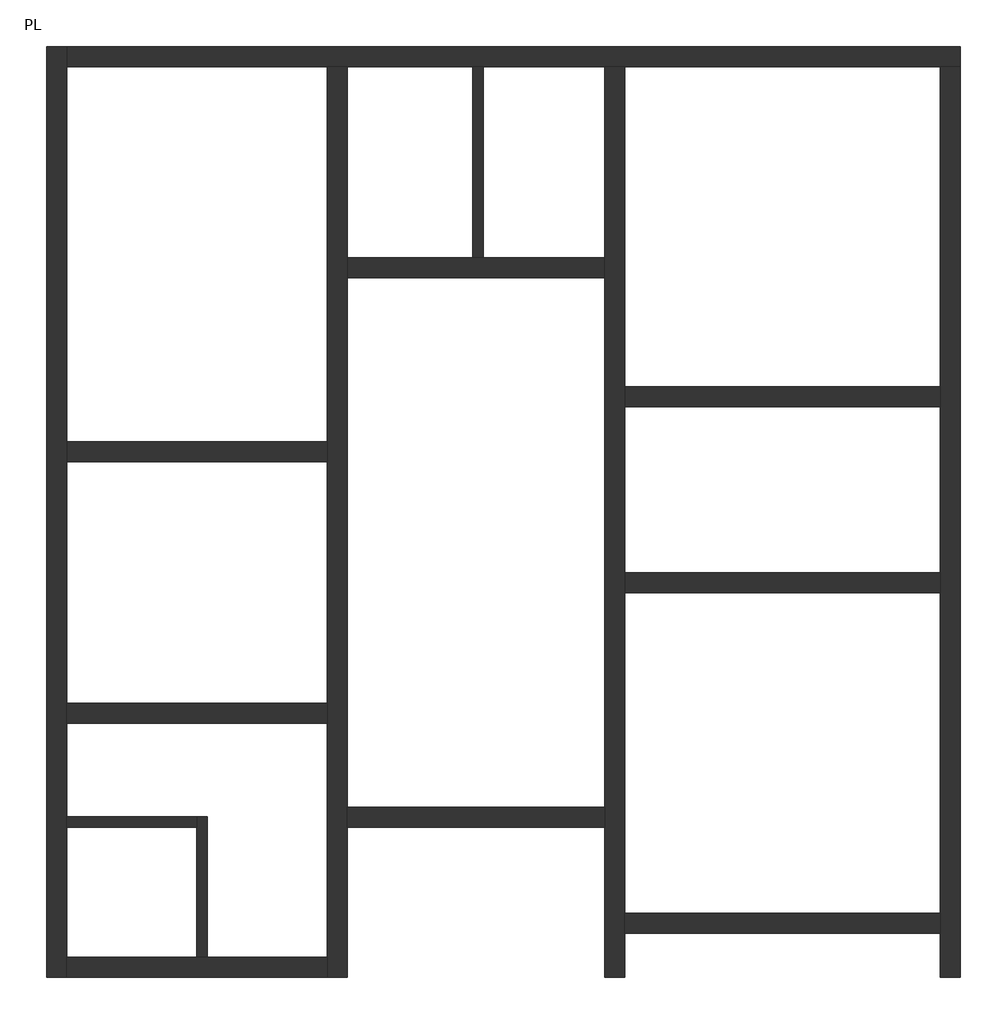
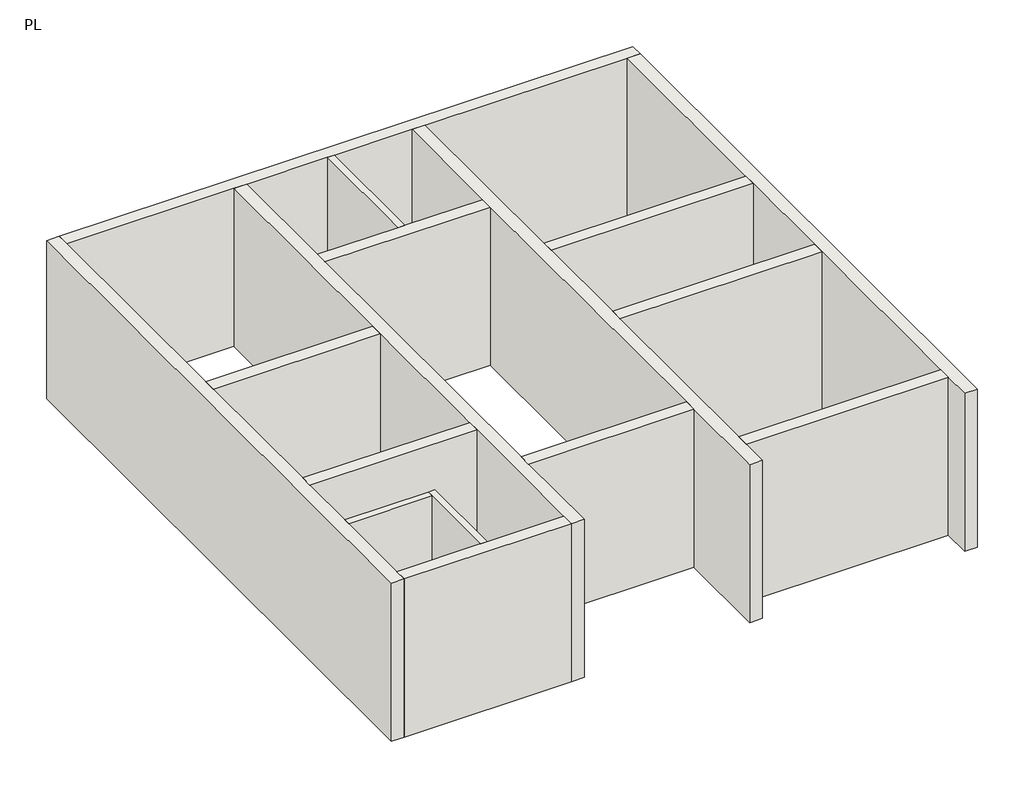
# One storey: 16 walls.
"""IFC4 building model written with IfcOpenShell, lengths in millimetres."""

from ifc_helpers import new_model, si_unit, frame, origin, place, context, project, spatial, polyline, outline, extrude, faceted_brep, element, save

model = new_model("IFC4")

# Units and contexts
model_context = context("Model", 3, world=origin())
ifc_project = project(units=[si_unit("LENGTHUNIT", "METRE", prefix="MILLI")], contexts=[model_context])

# Site, building, storey
site = spatial("IfcSite", under=ifc_project)
building = spatial("IfcBuilding", under=site)
storey = spatial("IfcBuildingStorey", under=building, Name="PL", Elevation=450.0)

# Walls
placement = place(None, origin())
element("IfcWall", 1, ObjectType="WALL 24", at=placement, inside=storey, context=model_context, shape_type="Brep", body=[
    faceted_brep([(-19136.5903863, 7865.0066114, 450.0), (-19136.5903863, -2854.9933886, 450.0), (-19136.5903863, -2854.9933886, 3450.0), (-19136.5903863, 7865.0066114, 3450.0), (-18906.5903863, 7865.0066114, 450.0), (-18906.5903863, 7865.0066114, 3450.0), (-18906.5903863, 7635.0066114, 3450.0), (-18906.5903863, 3315.0066114, 3450.0), (-18906.5903863, 3085.0066114, 3450.0), (-18906.5903863, 305.0066114, 3450.0), (-18906.5903863, 75.0066114, 3450.0), (-18906.5903863, -1004.9933886, 3450.0), (-18906.5903863, -1124.9933886, 3450.0), (-18906.5903863, -2624.9933886, 3450.0), (-18906.5903863, -2854.9933886, 3450.0), (-18906.5903863, -2854.9933886, 450.0), (-18906.5903863, -2624.9933886, 450.0), (-18906.5903863, -1124.9933886, 450.0), (-18906.5903863, -1004.9933886, 450.0), (-18906.5903863, 75.0066114, 450.0), (-18906.5903863, 305.0066114, 450.0), (-18906.5903863, 3085.0066114, 450.0), (-18906.5903863, 3315.0066114, 450.0), (-18906.5903863, 7635.0066114, 450.0)], [[[0, 1, 2, 3]], [[4, 5, 6, 7, 8, 9, 10, 11, 12, 13, 14, 15, 16, 17, 18, 19, 20, 21, 22, 23]], [[1, 0, 4, 23, 22, 21, 20, 19, 18, 17, 16, 15]], [[3, 2, 14, 13, 12, 11, 10, 9, 8, 7, 6, 5]], [[0, 3, 5, 4]], [[2, 1, 15, 14]]]),
])
element("IfcWall", 2, ObjectType="WALL 24", at=placement, inside=storey, context=model_context, shape_type="Brep", body=[
    faceted_brep([(-18906.5903863, 7635.0066114, 450.0), (-15906.5903863, 7635.0066114, 450.0), (-15676.5903863, 7635.0066114, 450.0), (-14226.5903863, 7635.0066114, 450.0), (-14106.5903863, 7635.0066114, 450.0), (-12706.5903863, 7635.0066114, 450.0), (-12476.5903863, 7635.0066114, 450.0), (-8846.5903863, 7635.0066114, 450.0), (-8616.5903863, 7635.0066114, 450.0), (-8616.5903863, 7635.0066114, 3450.0), (-8846.5903863, 7635.0066114, 3450.0), (-12476.5903863, 7635.0066114, 3450.0), (-12706.5903863, 7635.0066114, 3450.0), (-14106.5903863, 7635.0066114, 3450.0), (-14226.5903863, 7635.0066114, 3450.0), (-15676.5903863, 7635.0066114, 3450.0), (-15906.5903863, 7635.0066114, 3450.0), (-18906.5903863, 7635.0066114, 3450.0), (-18906.5903863, 7865.0066114, 450.0), (-18906.5903863, 7865.0066114, 3450.0), (-8616.5903863, 7865.0066114, 3450.0), (-8616.5903863, 7865.0066114, 450.0)], [[[0, 1, 2, 3, 4, 5, 6, 7, 8, 9, 10, 11, 12, 13, 14, 15, 16, 17]], [[18, 19, 20, 21]], [[8, 7, 6, 5, 4, 3, 2, 1, 0, 18, 21]], [[17, 16, 15, 14, 13, 12, 11, 10, 9, 20, 19]], [[0, 17, 19, 18]], [[9, 8, 21, 20]]]),
])
element("IfcWall", 3, ObjectType="WALL 24", at=placement, inside=storey, context=model_context, shape_type="Brep", body=[
    faceted_brep([(-15906.5903863, 7635.0066114, 450.0), (-15906.5903863, 3315.0066114, 450.0), (-15906.5903863, 3085.0066114, 450.0), (-15906.5903863, 305.0066114, 450.0), (-15906.5903863, 75.0066114, 450.0), (-15906.5903863, -2624.9933886, 450.0), (-15906.5903863, -2854.9933886, 450.0), (-15906.5903863, -2854.9933886, 3450.0), (-15906.5903863, -2624.9933886, 3450.0), (-15906.5903863, 75.0066114, 3450.0), (-15906.5903863, 305.0066114, 3450.0), (-15906.5903863, 3085.0066114, 3450.0), (-15906.5903863, 3315.0066114, 3450.0), (-15906.5903863, 7635.0066114, 3450.0), (-15676.5903863, 7635.0066114, 450.0), (-15676.5903863, 7635.0066114, 3450.0), (-15676.5903863, 5435.0066114, 3450.0), (-15676.5903863, 5205.0066114, 3450.0), (-15676.5903863, -894.9933886, 3450.0), (-15676.5903863, -1124.9933886, 3450.0), (-15676.5903863, -2854.9933886, 3450.0), (-15676.5903863, -2854.9933886, 450.0), (-15676.5903863, -1124.9933886, 450.0), (-15676.5903863, -894.9933886, 450.0), (-15676.5903863, 5205.0066114, 450.0), (-15676.5903863, 5435.0066114, 450.0)], [[[0, 1, 2, 3, 4, 5, 6, 7, 8, 9, 10, 11, 12, 13]], [[14, 15, 16, 17, 18, 19, 20, 21, 22, 23, 24, 25]], [[6, 5, 4, 3, 2, 1, 0, 14, 25, 24, 23, 22, 21]], [[13, 12, 11, 10, 9, 8, 7, 20, 19, 18, 17, 16, 15]], [[0, 13, 15, 14]], [[7, 6, 21, 20]]]),
])
element("IfcWall", 4, ObjectType="WALL 24", at=placement, inside=storey, context=model_context, shape_type="SweptSolid", body=[
    extrude(outline(polyline([(-18906.5903863, 3315.0066114), (-15906.5903863, 3315.0066114), (-15906.5903863, 3085.0066114), (-18906.5903863, 3085.0066114), (-18906.5903863, 3315.0066114)])), frame((0.0, 0.0, 450.0), z_axis=(0.0, 0.0, 1.0), x_axis=(1.0, 0.0, 0.0)), (0.0, 0.0, 1.0), 3000.0),
])
element("IfcWall", 5, ObjectType="WALL 24", at=placement, inside=storey, context=model_context, shape_type="SweptSolid", body=[
    extrude(outline(polyline([(-18906.5903863, 305.0066114), (-15906.5903863, 305.0066114), (-15906.5903863, 75.0066114), (-18906.5903863, 75.0066114), (-18906.5903863, 305.0066114)])), frame((0.0, 0.0, 450.0), z_axis=(0.0, 0.0, 1.0), x_axis=(1.0, 0.0, 0.0)), (0.0, 0.0, 1.0), 3000.0),
])
element("IfcWall", 6, ObjectType="WALL 24", at=placement, inside=storey, context=model_context, shape_type="Brep", body=[
    faceted_brep([(-15906.5903863, -2624.9933886, 450.0), (-17286.5903863, -2624.9933886, 450.0), (-17406.5903863, -2624.9933886, 450.0), (-18906.5903863, -2624.9933886, 450.0), (-18906.5903863, -2624.9933886, 3450.0), (-17406.5903863, -2624.9933886, 3450.0), (-17286.5903863, -2624.9933886, 3450.0), (-15906.5903863, -2624.9933886, 3450.0), (-15906.5903863, -2854.9933886, 450.0), (-15906.5903863, -2854.9933886, 3450.0), (-18906.5903863, -2854.9933886, 3450.0), (-18906.5903863, -2854.9933886, 450.0)], [[[0, 1, 2, 3, 4, 5, 6, 7]], [[8, 9, 10, 11]], [[3, 2, 1, 0, 8, 11]], [[7, 6, 5, 4, 10, 9]], [[4, 3, 11, 10]], [[0, 7, 9, 8]]]),
])
element("IfcWall", 7, ObjectType="WALL 24", at=placement, inside=storey, context=model_context, shape_type="Brep", body=[
    faceted_brep([(-12706.5903863, 7635.0066114, 450.0), (-12706.5903863, 5435.0066114, 450.0), (-12706.5903863, 5205.0066114, 450.0), (-12706.5903863, -894.9933886, 450.0), (-12706.5903863, -1124.9933886, 450.0), (-12706.5903863, -2854.9933886, 450.0), (-12706.5903863, -2854.9933886, 3450.0), (-12706.5903863, -1124.9933886, 3450.0), (-12706.5903863, -894.9933886, 3450.0), (-12706.5903863, 5205.0066114, 3450.0), (-12706.5903863, 5435.0066114, 3450.0), (-12706.5903863, 7635.0066114, 3450.0), (-12476.5903863, 7635.0066114, 450.0), (-12476.5903863, 7635.0066114, 3450.0), (-12476.5903863, 3945.0066114, 3450.0), (-12476.5903863, 3715.0066114, 3450.0), (-12476.5903863, 1805.0066114, 3450.0), (-12476.5903863, 1575.0066114, 3450.0), (-12476.5903863, -2114.9933886, 3450.0), (-12476.5903863, -2344.9933886, 3450.0), (-12476.5903863, -2854.9933886, 3450.0), (-12476.5903863, -2854.9933886, 450.0), (-12476.5903863, -2344.9933886, 450.0), (-12476.5903863, -2114.9933886, 450.0), (-12476.5903863, 1575.0066114, 450.0), (-12476.5903863, 1805.0066114, 450.0), (-12476.5903863, 3715.0066114, 450.0), (-12476.5903863, 3945.0066114, 450.0)], [[[0, 1, 2, 3, 4, 5, 6, 7, 8, 9, 10, 11]], [[12, 13, 14, 15, 16, 17, 18, 19, 20, 21, 22, 23, 24, 25, 26, 27]], [[5, 4, 3, 2, 1, 0, 12, 27, 26, 25, 24, 23, 22, 21]], [[6, 5, 21, 20]], [[11, 10, 9, 8, 7, 6, 20, 19, 18, 17, 16, 15, 14, 13]], [[0, 11, 13, 12]]]),
])
element("IfcWall", 8, ObjectType="WALL 24", at=placement, inside=storey, context=model_context, shape_type="Brep", body=[
    faceted_brep([(-8846.5903863, 7635.0066114, 450.0), (-8846.5903863, 3945.0066114, 450.0), (-8846.5903863, 3715.0066114, 450.0), (-8846.5903863, 1805.0066114, 450.0), (-8846.5903863, 1575.0066114, 450.0), (-8846.5903863, -2114.9933886, 450.0), (-8846.5903863, -2344.9933886, 450.0), (-8846.5903863, -2854.9933886, 450.0), (-8846.5903863, -2854.9933886, 3450.0), (-8846.5903863, -2344.9933886, 3450.0), (-8846.5903863, -2114.9933886, 3450.0), (-8846.5903863, 1575.0066114, 3450.0), (-8846.5903863, 1805.0066114, 3450.0), (-8846.5903863, 3715.0066114, 3450.0), (-8846.5903863, 3945.0066114, 3450.0), (-8846.5903863, 7635.0066114, 3450.0), (-8616.5903863, 7635.0066114, 450.0), (-8616.5903863, 7635.0066114, 3450.0), (-8616.5903863, -2854.9933886, 3450.0), (-8616.5903863, -2854.9933886, 450.0)], [[[0, 1, 2, 3, 4, 5, 6, 7, 8, 9, 10, 11, 12, 13, 14, 15]], [[16, 17, 18, 19]], [[7, 6, 5, 4, 3, 2, 1, 0, 16, 19]], [[8, 7, 19, 18]], [[15, 14, 13, 12, 11, 10, 9, 8, 18, 17]], [[0, 15, 17, 16]]]),
])
element("IfcWall", 9, ObjectType="WALL 24", at=placement, inside=storey, context=model_context, shape_type="SweptSolid", body=[
    extrude(outline(polyline([(-12476.5903863, 3945.0066114), (-8846.5903863, 3945.0066114), (-8846.5903863, 3715.0066114), (-12476.5903863, 3715.0066114), (-12476.5903863, 3945.0066114)])), frame((0.0, 0.0, 450.0), z_axis=(0.0, 0.0, 1.0), x_axis=(1.0, 0.0, 0.0)), (0.0, 0.0, 1.0), 3000.0),
])
element("IfcWall", 10, ObjectType="WALL 24", at=placement, inside=storey, context=model_context, shape_type="SweptSolid", body=[
    extrude(outline(polyline([(-12476.5903863, -2114.9933886), (-8846.5903863, -2114.9933886), (-8846.5903863, -2344.9933886), (-12476.5903863, -2344.9933886), (-12476.5903863, -2114.9933886)])), frame((0.0, 0.0, 450.0), z_axis=(0.0, 0.0, 1.0), x_axis=(1.0, 0.0, 0.0)), (0.0, 0.0, 1.0), 3000.0),
])
element("IfcWall", 11, ObjectType="WALL 24", at=placement, inside=storey, context=model_context, shape_type="SweptSolid", body=[
    extrude(outline(polyline([(-12706.5903863, -1124.9933886), (-15676.5903863, -1124.9933886), (-15676.5903863, -894.9933886), (-12706.5903863, -894.9933886), (-12706.5903863, -1124.9933886)])), frame((0.0, 0.0, 450.0), z_axis=(0.0, 0.0, 1.0), x_axis=(1.0, 0.0, 0.0)), (0.0, 0.0, 1.0), 3000.0),
])
element("IfcWall", 12, ObjectType="WALL 24", at=placement, inside=storey, context=model_context, shape_type="Brep", body=[
    faceted_brep([(-15676.5903863, 5205.0066114, 450.0), (-12706.5903863, 5205.0066114, 450.0), (-12706.5903863, 5205.0066114, 3450.0), (-15676.5903863, 5205.0066114, 3450.0), (-15676.5903863, 5435.0066114, 450.0), (-15676.5903863, 5435.0066114, 3450.0), (-14226.5903863, 5435.0066114, 3450.0), (-14106.5903863, 5435.0066114, 3450.0), (-12706.5903863, 5435.0066114, 3450.0), (-12706.5903863, 5435.0066114, 450.0), (-14106.5903863, 5435.0066114, 450.0), (-14226.5903863, 5435.0066114, 450.0)], [[[0, 1, 2, 3]], [[4, 5, 6, 7, 8, 9, 10, 11]], [[1, 0, 4, 11, 10, 9]], [[3, 2, 8, 7, 6, 5]], [[0, 3, 5, 4]], [[2, 1, 9, 8]]]),
])
element("IfcWall", 13, ObjectType="WALL 24", at=placement, inside=storey, context=model_context, shape_type="SweptSolid", body=[
    extrude(outline(polyline([(-8846.5903863, 1575.0066114), (-12476.5903863, 1575.0066114), (-12476.5903863, 1805.0066114), (-8846.5903863, 1805.0066114), (-8846.5903863, 1575.0066114)])), frame((0.0, 0.0, 450.0), z_axis=(0.0, 0.0, 1.0), x_axis=(1.0, 0.0, 0.0)), (0.0, 0.0, 1.0), 3000.0),
])
element("IfcWall", 14, ObjectType="WALL 25", at=placement, inside=storey, context=model_context, shape_type="SweptSolid", body=[
    extrude(outline(polyline([(-14226.5903863, 5435.0066114), (-14226.5903863, 7635.0066114), (-14106.5903863, 7635.0066114), (-14106.5903863, 5435.0066114), (-14226.5903863, 5435.0066114)])), frame((0.0, 0.0, 450.0), z_axis=(0.0, 0.0, 1.0), x_axis=(1.0, 0.0, 0.0)), (0.0, 0.0, 1.0), 3000.0),
])
element("IfcWall", 15, ObjectType="WALL 25", at=placement, inside=storey, context=model_context, shape_type="Brep", body=[
    faceted_brep([(-17286.5903863, -2624.9933886, 450.0), (-17286.5903863, -1004.9933886, 450.0), (-17286.5903863, -1004.9933886, 3450.0), (-17286.5903863, -2624.9933886, 3450.0), (-17406.5903863, -2624.9933886, 450.0), (-17406.5903863, -2624.9933886, 3450.0), (-17406.5903863, -1124.9933886, 3450.0), (-17406.5903863, -1004.9933886, 3450.0), (-17406.5903863, -1004.9933886, 450.0), (-17406.5903863, -1124.9933886, 450.0)], [[[0, 1, 2, 3]], [[4, 5, 6, 7, 8, 9]], [[1, 0, 4, 9, 8]], [[2, 1, 8, 7]], [[3, 2, 7, 6, 5]], [[0, 3, 5, 4]]]),
])
element("IfcWall", 16, ObjectType="WALL 25", at=placement, inside=storey, context=model_context, shape_type="SweptSolid", body=[
    extrude(outline(polyline([(-17406.5903863, -1124.9933886), (-18906.5903863, -1124.9933886), (-18906.5903863, -1004.9933886), (-17406.5903863, -1004.9933886), (-17406.5903863, -1124.9933886)])), frame((0.0, 0.0, 450.0), z_axis=(0.0, 0.0, 1.0), x_axis=(1.0, 0.0, 0.0)), (0.0, 0.0, 1.0), 3000.0),
])

save(model, "model.ifc")

# Revit data of these elements
# Project information
#   Project Issue Date = "Issue Date"
#   Project Status = "Project Status"
#   Client Name = "Owner"
#   Project Address = "Enter address here"
#   Project Name = "Project Name"
#   Project Number = "0001"
# Type "WALL 24"
#   Layers, outside or top first: 1.5 cm no material (function 4); 20 cm no material (function 1); 1.5 cm no material (function 5)
# Type "WALL 25"
#   Layers, outside or top first: 1.5 cm no material (function 4); 9 cm no material (function 1); 1.5 cm no material (function 5)
# Elements 1, 2, 3, 4, 5, 6, 7, 8, 9, 10, 11, 12, 13 (IfcWall, "WALL 24")
#   Top Offset = 0 cm
#   Base Offset = 0 cm
#   wall height = 300 cm
#   Phase Created = New Construction
#   Base Constraint = PL
#   Top Constraint = 1F
#   Materials on its faces: "Default Wall"
# Elements 14, 15, 16 (IfcWall, "WALL 25")
#   Top Offset = 0 cm
#   Base Offset = 0 cm
#   wall height = 300 cm
#   Phase Created = New Construction
#   Base Constraint = PL
#   Top Constraint = 1F
#   Materials on its faces: "Default Wall"
# Materials
#   "Default Wall": class "Miscellaneous", colour RGB 128 128 128, transparency 0, Cost = 0
